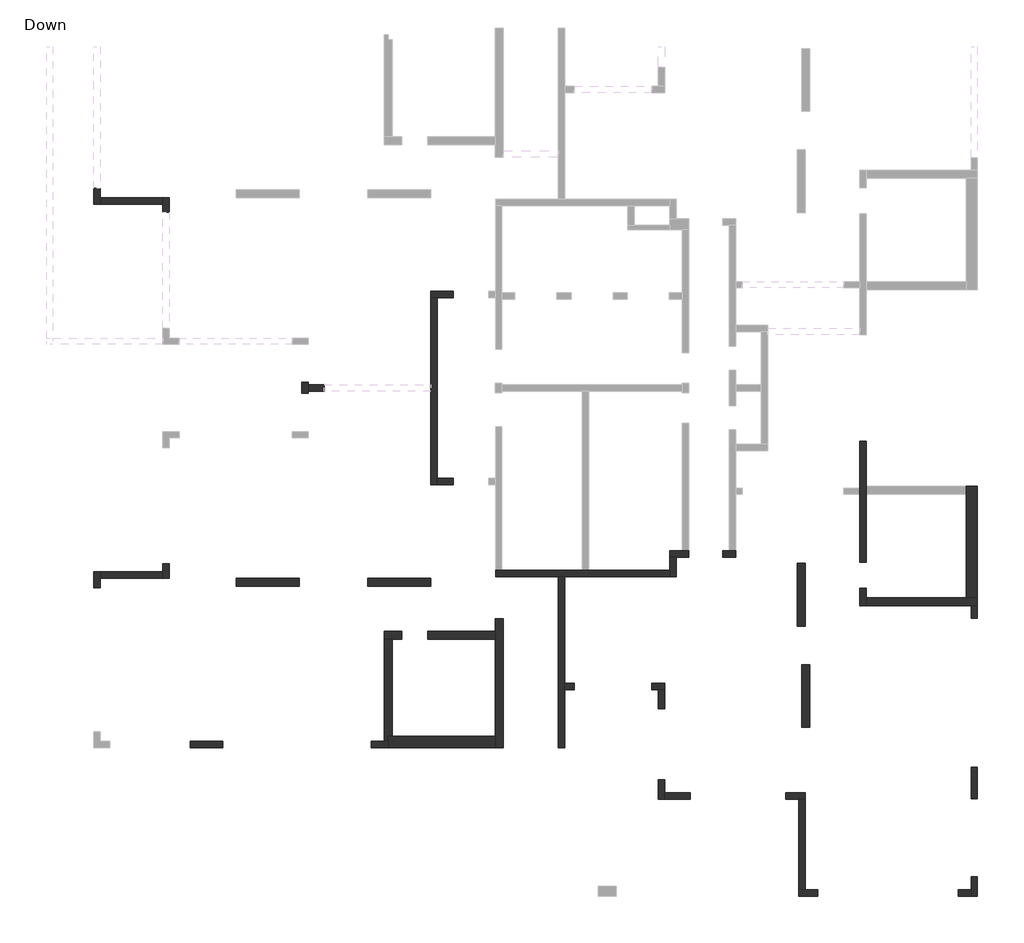
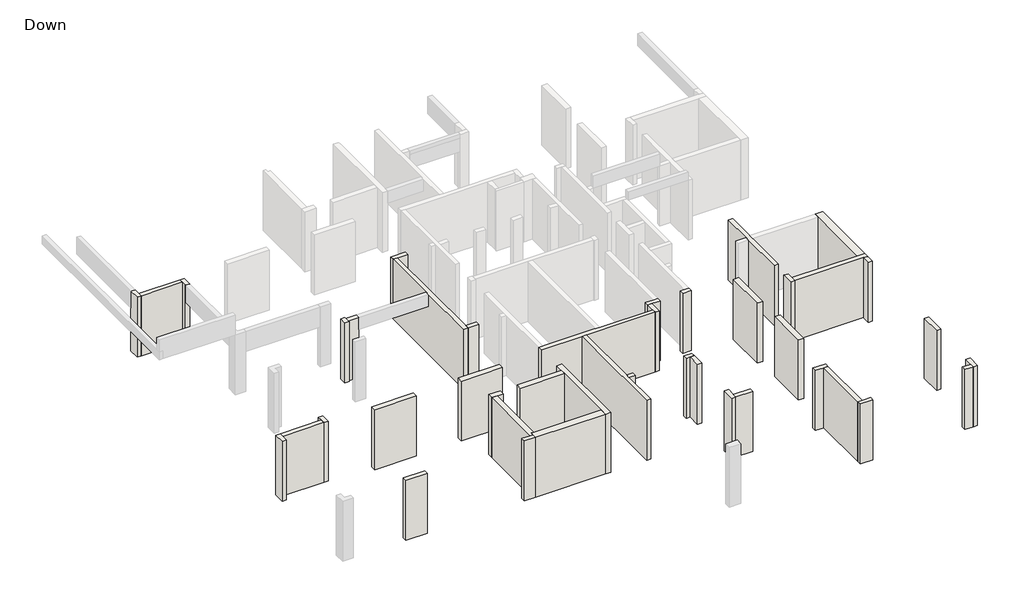
# One storey, part 1 of 3: 43 walls.
"""IFC4 building model written with IfcOpenShell, lengths in millimetres."""

from ifc_helpers import new_model, si_unit, origin, place, context, project, spatial, faceted_brep, element, save

model = new_model("IFC4")

# Units and contexts
model_context = context("Model", 3, world=origin())
ifc_project = project(units=[si_unit("LENGTHUNIT", "METRE", prefix="MILLI")], contexts=[model_context])

# Site, building, storey
site = spatial("IfcSite", under=ifc_project)
building = spatial("IfcBuilding", under=site)
storey = spatial("IfcBuildingStorey", under=building, Name="Down", Elevation=0.0)

# Walls
placement = place(None, origin())
element("IfcWall", 1, ObjectType="20", at=placement, inside=storey, context=model_context, shape_type="Brep", body=[
    faceted_brep([(-9805.5395337, 8939.7491377, 0.0), (-9805.5395337, 9386.8536298, 0.0), (-9805.5395337, 9386.8536298, 2820.0), (-9805.5395337, 9386.8536298, 3000.0), (-9805.5395337, 8939.7491377, 3000.0), (-9805.5395337, 8939.7491377, 2150.0), (-10005.5395337, 8939.7491377, 0.0), (-10005.5395337, 8939.7491377, 2150.0), (-10005.5395337, 8939.7491377, 3000.0), (-10005.5395337, 9186.8536298, 3000.0), (-10005.5395337, 9386.8536298, 3000.0), (-10005.5395337, 9386.8536298, 0.0), (-10005.5395337, 9186.8536298, 0.0)], [[[0, 1, 2, 3, 4, 5]], [[6, 7, 8, 9, 10, 11, 12]], [[1, 0, 6, 12, 11]], [[4, 3, 10, 9, 8]], [[0, 5, 4, 8, 7, 6]], [[3, 2, 1, 11, 10]]]),
])
element("IfcWall", 2, ObjectType="20", at=placement, inside=storey, context=model_context, shape_type="Brep", body=[
    faceted_brep([(-10005.5395337, 9386.8536298, 0.0), (-11954.2455884, 9386.8536298, 0.0), (-11954.2455884, 9386.8536298, 2820.0), (-11954.2455884, 9386.8536298, 3000.0), (-10005.5395337, 9386.8536298, 3000.0), (-10005.5395337, 9186.8536298, 0.0), (-10005.5395337, 9186.8536298, 2750.0), (-10005.5395337, 9186.8536298, 3000.0), (-11954.2455884, 9186.8536298, 3000.0), (-11954.2455884, 9186.8536298, 0.0)], [[[0, 1, 2, 3, 4]], [[5, 6, 7, 8, 9]], [[1, 0, 5, 9]], [[4, 3, 8, 7]], [[0, 4, 7, 6, 5]], [[3, 2, 1, 9, 8]]]),
])
element("IfcWall", 3, ObjectType="20", at=placement, inside=storey, context=model_context, shape_type="Brep", body=[
    faceted_brep([(-11954.2455884, 9186.8536298, 0.0), (-11954.2455884, 9386.8536298, 0.0), (-11954.2455884, 9686.3702314, 0.0), (-11954.2455884, 9686.3702314, 2150.0), (-11954.2455884, 9686.3702314, 3000.0), (-11954.2455884, 9386.8536298, 3000.0), (-11954.2455884, 9186.8536298, 3000.0), (-12154.2455884, 9186.8536298, 0.0), (-12154.2455884, 9186.8536298, 2750.0), (-12154.2455884, 9186.8536298, 3000.0), (-12154.2455884, 9686.3702314, 3000.0), (-12154.2455884, 9686.3702314, 2150.0), (-12154.2455884, 9686.3702314, 0.0)], [[[0, 1, 2, 3, 4, 5, 6]], [[7, 8, 9, 10, 11, 12]], [[2, 1, 0, 7, 12]], [[4, 3, 2, 12, 11, 10]], [[6, 5, 4, 10, 9]], [[0, 6, 9, 8, 7]]]),
])
element("IfcWall", 4, ObjectType="20", at=placement, inside=storey, context=model_context, shape_type="Brep", body=[
    faceted_brep([(-1004.8486157, 6491.5264814, 0.0), (-1704.8486157, 6491.5264814, 0.0), (-1704.8486157, 6491.5264814, 2820.0), (-1704.8486157, 6491.5264814, 3000.0), (-1004.8486157, 6491.5264814, 3000.0), (-1004.8486157, 6491.5264814, 2820.0), (-1004.8486157, 6291.5264814, 0.0), (-1004.8486157, 6291.5264814, 2820.0), (-1004.8486157, 6291.5264814, 3000.0), (-1504.8486157, 6291.5264814, 3000.0), (-1704.8486157, 6291.5264814, 3000.0), (-1704.8486157, 6291.5264814, 0.0), (-1504.8486157, 6291.5264814, 0.0)], [[[0, 1, 2, 3, 4, 5]], [[6, 7, 8, 9, 10, 11, 12]], [[1, 0, 6, 12, 11]], [[4, 3, 10, 9, 8]], [[0, 5, 4, 8, 7, 6]], [[3, 2, 1, 11, 10]]]),
])
element("IfcWall", 5, ObjectType="20", at=placement, inside=storey, context=model_context, shape_type="Brep", body=[
    faceted_brep([(-1704.8486157, 6291.5264814, 0.0), (-1704.8486157, 491.1895673, 0.0), (-1704.8486157, 491.1895673, 2820.0), (-1704.8486157, 491.1895673, 3000.0), (-1704.8486157, 3390.0103681, 3000.0), (-1704.8486157, 3590.0103681, 3000.0), (-1704.8486157, 6291.5264814, 3000.0), (-1504.8486157, 6291.5264814, 0.0), (-1504.8486157, 6291.5264814, 2820.0), (-1504.8486157, 6291.5264814, 3000.0), (-1504.8486157, 691.1895673, 3000.0), (-1504.8486157, 491.1895673, 3000.0), (-1504.8486157, 491.1895673, 0.0), (-1504.8486157, 691.1895673, 0.0)], [[[0, 1, 2, 3, 4, 5, 6]], [[7, 8, 9, 10, 11, 12, 13]], [[1, 0, 7, 13, 12]], [[6, 5, 4, 3, 11, 10, 9]], [[0, 6, 9, 8, 7]], [[3, 2, 1, 12, 11]]]),
])
element("IfcWall", 6, ObjectType="20", at=placement, inside=storey, context=model_context, shape_type="Brep", body=[
    faceted_brep([(-1504.8486157, 491.1895673, 0.0), (-999.8486157, 491.1895673, 0.0), (-999.8486157, 491.1895673, 2820.0), (-999.8486157, 491.1895673, 3000.0), (-1504.8486157, 491.1895673, 3000.0), (-1504.8486157, 691.1895673, 0.0), (-1504.8486157, 691.1895673, 2820.0), (-1504.8486157, 691.1895673, 3000.0), (-999.8486157, 691.1895673, 3000.0), (-999.8486157, 691.1895673, 2820.0), (-999.8486157, 691.1895673, 0.0), (-999.8486157, 688.4942548, 3000.0)], [[[0, 1, 2, 3, 4]], [[5, 6, 7, 8, 9, 10]], [[1, 0, 5, 10]], [[3, 2, 1, 10, 9, 8, 11]], [[4, 3, 11, 8, 7]], [[0, 4, 7, 6, 5]]]),
])
element("IfcWall", 7, ObjectType="20", at=placement, inside=storey, context=model_context, shape_type="Brep", body=[
    faceted_brep([(-5499.4457837, 3320.5572431, 0.0), (-5499.4457837, 3390.0103681, 0.0), (-5499.4457837, 3590.0103681, 0.0), (-5499.4457837, 3661.3116377, 0.0), (-5499.4457837, 3661.3116377, 3000.0), (-5499.4457837, 3590.0103681, 3000.0), (-5499.4457837, 3390.0103681, 3000.0), (-5499.4457837, 3320.5572431, 3000.0), (-5699.4457837, 3320.5572431, 0.0), (-5699.4457837, 3320.5572431, 3000.0), (-5699.4457837, 3661.3116377, 3000.0), (-5699.4457837, 3661.3116377, 0.0)], [[[0, 1, 2, 3, 4, 5, 6, 7]], [[8, 9, 10, 11]], [[3, 2, 1, 0, 8, 11]], [[4, 3, 11, 10]], [[7, 6, 5, 4, 10, 9]], [[0, 7, 9, 8]]]),
])
element("IfcWall", 8, ObjectType="20", at=placement, inside=storey, context=model_context, shape_type="Brep", body=[
    faceted_brep([(-5004.9145337, 3590.0103681, 0.0), (-5499.4457837, 3590.0103681, 0.0), (-5499.4457837, 3590.0103681, 2820.0), (-5499.4457837, 3590.0103681, 3000.0), (-5004.9145337, 3590.0103681, 3000.0), (-5004.9145337, 3590.0103681, 2400.0), (-5004.9145337, 3390.0103681, 0.0), (-5004.9145337, 3390.0103681, 2400.0), (-5004.9145337, 3390.0103681, 3000.0), (-5499.4457837, 3390.0103681, 3000.0), (-5499.4457837, 3390.0103681, 2820.0), (-5499.4457837, 3390.0103681, 0.0)], [[[0, 1, 2, 3, 4, 5]], [[6, 7, 8, 9, 10, 11]], [[1, 0, 6, 11]], [[4, 3, 9, 8]], [[0, 5, 4, 8, 7, 6]], [[3, 2, 1, 11, 10, 9]]]),
])
element("IfcWall", 9, ObjectType="20", at=placement, inside=storey, context=model_context, shape_type="Brep", body=[
    faceted_brep([(-10005.5395337, -1959.7284014, 0.0), (-10005.5395337, -2206.8328936, 0.0), (-10005.5395337, -2406.8328936, 0.0), (-10005.5395337, -2406.8328936, 3000.0), (-10005.5395337, -2206.8328936, 3000.0), (-10005.5395337, -1959.7284014, 3000.0), (-10005.5395337, -1959.7284014, 2150.0), (-9805.5395337, -1959.7284014, 0.0), (-9805.5395337, -1959.7284014, 2150.0), (-9805.5395337, -1959.7284014, 3000.0), (-9805.5395337, -2406.8328936, 3000.0), (-9805.5395337, -2406.8328936, 2820.0), (-9805.5395337, -2406.8328936, 0.0)], [[[0, 1, 2, 3, 4, 5, 6]], [[7, 8, 9, 10, 11, 12]], [[2, 1, 0, 7, 12]], [[5, 4, 3, 10, 9]], [[0, 6, 5, 9, 8, 7]], [[3, 2, 12, 11, 10]]]),
])
element("IfcWall", 10, ObjectType="20", at=placement, inside=storey, context=model_context, shape_type="Brep", body=[
    faceted_brep([(-10005.5395337, -2206.8328936, 0.0), (-11954.2455884, -2206.8328936, 0.0), (-11954.2455884, -2206.8328936, 3000.0), (-10005.5395337, -2206.8328936, 3000.0), (-10005.5395337, -2206.8328936, 2750.0), (-10005.5395337, -2406.8328936, 0.0), (-10005.5395337, -2406.8328936, 3000.0), (-11954.2455884, -2406.8328936, 3000.0), (-11954.2455884, -2406.8328936, 2820.0), (-11954.2455884, -2406.8328936, 0.0)], [[[0, 1, 2, 3, 4]], [[5, 6, 7, 8, 9]], [[1, 0, 5, 9]], [[3, 2, 7, 6]], [[0, 4, 3, 6, 5]], [[2, 1, 9, 8, 7]]]),
])
element("IfcWall", 11, ObjectType="20", at=placement, inside=storey, context=model_context, shape_type="Brep", body=[
    faceted_brep([(-12154.2455884, -2206.8328936, 0.0), (-12154.2455884, -2706.3494952, 0.0), (-12154.2455884, -2706.3494952, 2150.0), (-12154.2455884, -2706.3494952, 3000.0), (-12154.2455884, -2206.8328936, 3000.0), (-12154.2455884, -2206.8328936, 2750.0), (-11954.2455884, -2206.8328936, 0.0), (-11954.2455884, -2206.8328936, 3000.0), (-11954.2455884, -2406.8328936, 3000.0), (-11954.2455884, -2706.3494952, 3000.0), (-11954.2455884, -2706.3494952, 2150.0), (-11954.2455884, -2706.3494952, 0.0), (-11954.2455884, -2406.8328936, 0.0)], [[[0, 1, 2, 3, 4, 5]], [[6, 7, 8, 9, 10, 11, 12]], [[1, 0, 6, 12, 11]], [[3, 2, 1, 11, 10, 9]], [[4, 3, 9, 8, 7]], [[0, 5, 4, 7, 6]]]),
])
element("IfcWall", 12, ObjectType="20", at=placement, inside=storey, context=model_context, shape_type="Brep", body=[
    faceted_brep([(-3022.0483227, -7461.3958819, 0.0), (-3147.0483227, -7461.3958819, 0.0), (-3547.0483227, -7461.3958819, 0.0), (-3547.0483227, -7461.3958819, 2450.0), (-3547.0483227, -7461.3958819, 2820.0), (-3547.0483227, -7461.3958819, 3000.0), (-3147.0483227, -7461.3958819, 3000.0), (-3022.0483227, -7461.3958819, 3000.0), (-3022.0483227, -7661.3958819, 0.0), (-3022.0483227, -7661.3958819, 3000.0), (-3547.0483227, -7661.3958819, 3000.0), (-3547.0483227, -7661.3958819, 2450.0), (-3547.0483227, -7661.3958819, 0.0), (-3547.0483227, -7466.3958819, 3000.0)], [[[0, 1, 2, 3, 4, 5, 6, 7]], [[8, 9, 10, 11, 12]], [[2, 1, 0, 8, 12]], [[5, 4, 3, 2, 12, 11, 10, 13]], [[7, 6, 5, 13, 10, 9]], [[0, 7, 9, 8]]]),
])
element("IfcWall", 13, ObjectType="20", at=placement, inside=storey, context=model_context, shape_type="Brep", body=[
    faceted_brep([(-9154.7387524, -7661.3958819, 0.0), (-8149.7387524, -7661.3958819, 0.0), (-8149.7387524, -7661.3958819, 2450.0), (-8149.7387524, -7661.3958819, 3000.0), (-9154.7387524, -7661.3958819, 3000.0), (-9154.7387524, -7661.3958819, 2450.0), (-9154.7387524, -7461.3958819, 0.0), (-9154.7387524, -7461.3958819, 2450.0), (-9154.7387524, -7461.3958819, 2820.0), (-9154.7387524, -7461.3958819, 3000.0), (-8149.7387524, -7461.3958819, 3000.0), (-8149.7387524, -7461.3958819, 2820.0), (-8149.7387524, -7461.3958819, 2450.0), (-8149.7387524, -7461.3958819, 0.0), (-8149.7387524, -7466.3958819, 3000.0), (-9154.7387524, -7466.3958819, 3000.0)], [[[0, 1, 2, 3, 4, 5]], [[6, 7, 8, 9, 10, 11, 12, 13]], [[1, 0, 6, 13]], [[3, 2, 1, 13, 12, 11, 10, 14]], [[4, 3, 14, 10, 9, 15]], [[0, 5, 4, 15, 9, 8, 7, 6]]]),
])
element("IfcWall", 14, ObjectType="20", at=placement, inside=storey, context=model_context, shape_type="Brep", body=[
    faceted_brep([(2446.4257984, -7661.3958819, 0.0), (2446.4257984, -5860.2777178, 0.0), (2446.4257984, -5660.2777178, 0.0), (2446.4257984, -2357.0550616, 0.0), (2446.4257984, -2357.0550616, 2820.0), (2446.4257984, -2357.0550616, 3000.0), (2446.4257984, -5660.2777178, 3000.0), (2446.4257984, -5860.2777178, 3000.0), (2446.4257984, -7661.3958819, 3000.0), (2446.4257984, -7661.3958819, 2750.0), (2246.4257984, -7661.3958819, 0.0), (2246.4257984, -7661.3958819, 2750.0), (2246.4257984, -7661.3958819, 3000.0), (2246.4257984, -7461.3958819, 3000.0), (2246.4257984, -3861.3299639, 3000.0), (2246.4257984, -3661.3299639, 3000.0), (2246.4257984, -2357.0550616, 3000.0), (2246.4257984, -2357.0550616, 2820.0), (2246.4257984, -2357.0550616, 0.0)], [[[0, 1, 2, 3, 4, 5, 6, 7, 8, 9]], [[10, 11, 12, 13, 14, 15, 16, 17, 18]], [[3, 2, 1, 0, 10, 18]], [[8, 7, 6, 5, 16, 15, 14, 13, 12]], [[0, 9, 8, 12, 11, 10]], [[5, 4, 3, 18, 17, 16]]]),
])
element("IfcWall", 15, ObjectType="20", at=placement, inside=storey, context=model_context, shape_type="Brep", body=[
    faceted_brep([(2745.6201343, -5660.2777178, 0.0), (2446.4257984, -5660.2777178, 0.0), (2446.4257984, -5660.2777178, 2820.0), (2446.4257984, -5660.2777178, 3000.0), (2745.6201343, -5660.2777178, 3000.0), (2745.6201343, -5660.2777178, 2820.0), (2745.6201343, -5660.2777178, 2150.0), (2745.6201343, -5860.2777178, 0.0), (2745.6201343, -5860.2777178, 2150.0), (2745.6201343, -5860.2777178, 3000.0), (2446.4257984, -5860.2777178, 3000.0), (2446.4257984, -5860.2777178, 0.0), (2745.6201343, -5665.2777178, 3000.0)], [[[0, 1, 2, 3, 4, 5, 6]], [[7, 8, 9, 10, 11]], [[1, 0, 7, 11]], [[4, 3, 10, 9, 12]], [[0, 6, 5, 4, 12, 9, 8, 7]], [[3, 2, 1, 11, 10]]]),
])
element("IfcWall", 16, ObjectType="20", at=placement, inside=storey, context=model_context, shape_type="Brep", body=[
    faceted_brep([(5152.6049976, -5860.2777178, 0.0), (5345.4492359, -5860.2777178, 0.0), (5545.4492359, -5860.2777178, 0.0), (5545.4492359, -5860.2777178, 3000.0), (5345.4492359, -5860.2777178, 3000.0), (5152.6049976, -5860.2777178, 3000.0), (5152.6049976, -5860.2777178, 2150.0), (5152.6049976, -5660.2777178, 0.0), (5152.6049976, -5660.2777178, 2150.0), (5152.6049976, -5660.2777178, 2820.0), (5152.6049976, -5660.2777178, 3000.0), (5545.4492359, -5660.2777178, 3000.0), (5545.4492359, -5660.2777178, 2820.0), (5545.4492359, -5660.2777178, 0.0), (5152.6049976, -5665.2777178, 3000.0)], [[[0, 1, 2, 3, 4, 5, 6]], [[7, 8, 9, 10, 11, 12, 13]], [[2, 1, 0, 7, 13]], [[5, 4, 3, 11, 10, 14]], [[0, 6, 5, 14, 10, 9, 8, 7]], [[3, 2, 13, 12, 11]]]),
])
element("IfcWall", 17, ObjectType="20", at=placement, inside=storey, context=model_context, shape_type="Brep", body=[
    faceted_brep([(5345.4492359, -5860.2777178, 0.0), (5345.4492359, -6456.8182452, 0.0), (5345.4492359, -6456.8182452, 2150.0), (5345.4492359, -6456.8182452, 3000.0), (5345.4492359, -5860.2777178, 3000.0), (5345.4492359, -5860.2777178, 2750.0), (5545.4492359, -5860.2777178, 0.0), (5545.4492359, -5860.2777178, 3000.0), (5545.4492359, -6456.8182452, 3000.0), (5545.4492359, -6456.8182452, 2150.0), (5545.4492359, -6456.8182452, 0.0)], [[[0, 1, 2, 3, 4, 5]], [[6, 7, 8, 9, 10]], [[1, 0, 6, 10]], [[3, 2, 1, 10, 9, 8]], [[4, 3, 8, 7]], [[0, 5, 4, 7, 6]]]),
])
element("IfcWall", 18, ObjectType="20", at=placement, inside=storey, context=model_context, shape_type="Brep", body=[
    faceted_brep([(5345.4492359, -8661.9549639, 0.0), (5345.4492359, -9261.9549639, 0.0), (5345.4492359, -9261.9549639, 2750.0), (5345.4492359, -9261.9549639, 3000.0), (5345.4492359, -8661.9549639, 3000.0), (5345.4492359, -8661.9549639, 2150.0), (5545.4492359, -8661.9549639, 0.0), (5545.4492359, -8661.9549639, 2150.0), (5545.4492359, -8661.9549639, 3000.0), (5545.4492359, -9061.9549639, 3000.0), (5545.4492359, -9261.9549639, 3000.0), (5545.4492359, -9261.9549639, 0.0), (5545.4492359, -9061.9549639, 0.0)], [[[0, 1, 2, 3, 4, 5]], [[6, 7, 8, 9, 10, 11, 12]], [[1, 0, 6, 12, 11]], [[4, 3, 10, 9, 8]], [[0, 5, 4, 8, 7, 6]], [[3, 2, 1, 11, 10]]]),
])
element("IfcWall", 19, ObjectType="20", at=placement, inside=storey, context=model_context, shape_type="Brep", body=[
    faceted_brep([(5545.4492359, -9261.9549639, 0.0), (6350.1123218, -9261.9549639, 0.0), (6350.1123218, -9261.9549639, 2150.0), (6350.1123218, -9261.9549639, 3000.0), (5545.4492359, -9261.9549639, 3000.0), (5545.4492359, -9061.9549639, 0.0), (5545.4492359, -9061.9549639, 2820.0), (5545.4492359, -9061.9549639, 3000.0), (6350.1123218, -9061.9549639, 3000.0), (6350.1123218, -9061.9549639, 2150.0), (6350.1123218, -9061.9549639, 0.0)], [[[0, 1, 2, 3, 4]], [[5, 6, 7, 8, 9, 10]], [[1, 0, 5, 10]], [[3, 2, 1, 10, 9, 8]], [[4, 3, 8, 7]], [[0, 4, 7, 6, 5]]]),
])
element("IfcWall", 20, ObjectType="20", at=placement, inside=storey, context=model_context, shape_type="Brep", body=[
    faceted_brep([(9302.4292163, -9261.9354327, 0.0), (9702.4292163, -9261.9354327, 0.0), (9902.4292163, -9261.9354327, 0.0), (9902.4292163, -9261.9354327, 3000.0), (9702.4292163, -9261.9354327, 3000.0), (9302.4292163, -9261.9354327, 3000.0), (9302.4292163, -9061.9354327, 0.0), (9302.4292163, -9061.9354327, 3000.0), (9902.4292163, -9061.9354327, 3000.0), (9902.4292163, -9061.9354327, 2820.0), (9902.4292163, -9061.9354327, 0.0)], [[[0, 1, 2, 3, 4, 5]], [[6, 7, 8, 9, 10]], [[2, 1, 0, 6, 10]], [[5, 4, 3, 8, 7]], [[0, 5, 7, 6]], [[3, 2, 10, 9, 8]]]),
])
element("IfcWall", 21, ObjectType="20", at=placement, inside=storey, context=model_context, shape_type="Brep", body=[
    faceted_brep([(9702.4292163, -9261.9354327, 0.0), (9702.4292163, -12061.3104327, 0.0), (9702.4292163, -12061.3104327, 3000.0), (9702.4292163, -9261.9354327, 3000.0), (9702.4292163, -9261.9354327, 2750.0), (9902.4292163, -9261.9354327, 0.0), (9902.4292163, -9261.9354327, 3000.0), (9902.4292163, -12061.3104327, 3000.0), (9902.4292163, -12061.3104327, 2820.0), (9902.4292163, -12061.3104327, 0.0)], [[[0, 1, 2, 3, 4]], [[5, 6, 7, 8, 9]], [[1, 0, 5, 9]], [[3, 2, 7, 6]], [[0, 4, 3, 6, 5]], [[2, 1, 9, 8, 7]]]),
])
element("IfcWall", 22, ObjectType="20", at=placement, inside=storey, context=model_context, shape_type="Brep", body=[
    faceted_brep([(9702.4292163, -12261.3104327, 0.0), (10302.4292163, -12261.3104327, 0.0), (10302.4292163, -12261.3104327, 2400.0), (10302.4292163, -12261.3104327, 3000.0), (9702.4292163, -12261.3104327, 3000.0), (9702.4292163, -12261.3104327, 2750.0), (9702.4292163, -12061.3104327, 0.0), (9702.4292163, -12061.3104327, 3000.0), (9902.4292163, -12061.3104327, 3000.0), (10302.4292163, -12061.3104327, 3000.0), (10302.4292163, -12061.3104327, 2820.0), (10302.4292163, -12061.3104327, 2400.0), (10302.4292163, -12061.3104327, 0.0), (9902.4292163, -12061.3104327, 0.0), (10302.4292163, -12066.3104327, 3000.0)], [[[0, 1, 2, 3, 4, 5]], [[6, 7, 8, 9, 10, 11, 12, 13]], [[1, 0, 6, 13, 12]], [[3, 2, 1, 12, 11, 10, 9, 14]], [[4, 3, 14, 9, 8, 7]], [[0, 5, 4, 7, 6]]]),
])
element("IfcWall", 23, ObjectType="20", at=placement, inside=storey, context=model_context, shape_type="Brep", body=[
    faceted_brep([(14652.4902515, -12261.3104327, 0.0), (15047.1826343, -12261.3104327, 0.0), (15047.1826343, -12261.3104327, 3000.0), (14652.4902515, -12261.3104327, 3000.0), (14652.4902515, -12261.3104327, 2400.0), (14652.4902515, -12061.3104327, 0.0), (14652.4902515, -12061.3104327, 2400.0), (14652.4902515, -12061.3104327, 2820.0), (14652.4902515, -12061.3104327, 3000.0), (15047.1826343, -12061.3104327, 3000.0), (15047.1826343, -12061.3104327, 2820.0), (15047.1826343, -12061.3104327, 0.0), (14652.4902515, -12066.3104327, 3000.0)], [[[0, 1, 2, 3, 4]], [[5, 6, 7, 8, 9, 10, 11]], [[1, 0, 5, 11]], [[3, 2, 9, 8, 12]], [[0, 4, 3, 12, 8, 7, 6, 5]], [[2, 1, 11, 10, 9]]]),
])
element("IfcWall", 24, ObjectType="20", at=placement, inside=storey, context=model_context, shape_type="Brep", body=[
    faceted_brep([(15247.1826343, -12261.3104327, 0.0), (15247.1826343, -11661.3104327, 0.0), (15247.1826343, -11661.3104327, 2400.0), (15247.1826343, -11661.3104327, 3000.0), (15247.1826343, -12261.3104327, 3000.0), (15047.1826343, -12261.3104327, 0.0), (15047.1826343, -12261.3104327, 3000.0), (15047.1826343, -12061.3104327, 3000.0), (15047.1826343, -11661.3104327, 3000.0), (15047.1826343, -11661.3104327, 2400.0), (15047.1826343, -11661.3104327, 0.0), (15047.1826343, -12061.3104327, 0.0)], [[[0, 1, 2, 3, 4]], [[5, 6, 7, 8, 9, 10, 11]], [[1, 0, 5, 11, 10]], [[3, 2, 1, 10, 9, 8]], [[4, 3, 8, 7, 6]], [[0, 4, 6, 5]]]),
])
element("IfcWall", 25, ObjectType="20", at=placement, inside=storey, context=model_context, shape_type="Brep", body=[
    faceted_brep([(15247.1826343, -9252.3065264, 0.0), (15247.1826343, -8260.429085, 0.0), (15247.1826343, -8260.429085, 2400.0), (15247.1826343, -8260.429085, 3000.0), (15247.1826343, -9252.3065264, 3000.0), (15247.1826343, -9252.3065264, 2400.0), (15047.1826343, -9252.3065264, 0.0), (15047.1826343, -9252.3065264, 2400.0), (15047.1826343, -9252.3065264, 3000.0), (15047.1826343, -8260.429085, 3000.0), (15047.1826343, -8260.429085, 2400.0), (15047.1826343, -8260.429085, 0.0)], [[[0, 1, 2, 3, 4, 5]], [[6, 7, 8, 9, 10, 11]], [[1, 0, 6, 11]], [[3, 2, 1, 11, 10, 9]], [[4, 3, 9, 8]], [[0, 5, 4, 8, 7, 6]]]),
])
element("IfcWall", 26, ObjectType="20", at=placement, inside=storey, context=model_context, shape_type="Brep", body=[
    faceted_brep([(15247.1826343, -3654.8187334, 0.0), (15247.1826343, -3259.804085, 0.0), (15247.1826343, -3259.804085, 3000.0), (15247.1826343, -3654.8187334, 3000.0), (15247.1826343, -3654.8187334, 2400.0), (15047.1826343, -3654.8187334, 0.0), (15047.1826343, -3654.8187334, 2400.0), (15047.1826343, -3654.8187334, 3000.0), (15047.1826343, -3259.804085, 3000.0), (15047.1826343, -3259.804085, 0.0)], [[[0, 1, 2, 3, 4]], [[5, 6, 7, 8, 9]], [[1, 0, 5, 9]], [[3, 2, 8, 7]], [[0, 4, 3, 7, 6, 5]], [[2, 1, 9, 8]]]),
])
element("IfcWall", 27, ObjectType="20", at=placement, inside=storey, context=model_context, shape_type="Brep", body=[
    faceted_brep([(11796.5527515, -3259.804085, 0.0), (11796.5527515, -3009.804085, 0.0), (11796.5527515, -2710.6903155, 0.0), (11796.5527515, -2710.6903155, 3000.0), (11796.5527515, -3009.804085, 3000.0), (11796.5527515, -3259.804085, 3000.0), (11596.5527515, -3259.804085, 0.0), (11596.5527515, -3259.804085, 2820.0), (11596.5527515, -3259.804085, 3000.0), (11596.5527515, -2710.6903155, 3000.0), (11596.5527515, -2710.6903155, 0.0)], [[[0, 1, 2, 3, 4, 5]], [[6, 7, 8, 9, 10]], [[2, 1, 0, 6, 10]], [[3, 2, 10, 9]], [[5, 4, 3, 9, 8]], [[0, 5, 8, 7, 6]]]),
])
element("IfcWall", 28, ObjectType="20", at=placement, inside=storey, context=model_context, shape_type="Brep", body=[
    faceted_brep([(11796.5527515, -1909.8089678, 0.0), (11796.5527515, 188.5748212, 0.0), (11796.5527515, 438.5748212, 0.0), (11796.5527515, 1845.1910322, 0.0), (11796.5527515, 1845.1910322, 3000.0), (11796.5527515, 438.5748212, 3000.0), (11796.5527515, 188.5748212, 3000.0), (11796.5527515, -1909.8089678, 3000.0), (11796.5527515, -1909.8089678, 2820.0), (11596.5527515, -1909.8089678, 0.0), (11596.5527515, -1909.8089678, 2820.0), (11596.5527515, -1909.8089678, 3000.0), (11596.5527515, 188.6553877, 3000.0), (11596.5527515, 388.6553877, 3000.0), (11596.5527515, 1845.1910322, 3000.0), (11596.5527515, 1845.1910322, 2820.0), (11596.5527515, 1845.1910322, 0.0), (11596.5527515, 388.6553877, 0.0), (11596.5527515, 188.6553877, 0.0)], [[[0, 1, 2, 3, 4, 5, 6, 7, 8]], [[9, 10, 11, 12, 13, 14, 15, 16, 17, 18]], [[3, 2, 1, 0, 9, 18, 17, 16]], [[4, 3, 16, 15, 14]], [[7, 6, 5, 4, 14, 13, 12, 11]], [[0, 8, 7, 11, 10, 9]]]),
])
element("IfcWall", 29, ObjectType="20", at=placement, inside=storey, context=model_context, shape_type="Brep", body=[
    faceted_brep([(5901.4257984, -2357.0550616, 0.0), (5901.4257984, -1759.7284014, 0.0), (5901.4257984, -1759.7284014, 2820.0), (5901.4257984, -1759.7284014, 3000.0), (5901.4257984, -2357.0550616, 3000.0), (5901.4257984, -2357.0550616, 2820.0), (5701.4257984, -2357.0550616, 0.0), (5701.4257984, -2357.0550616, 3000.0), (5701.4257984, -2157.0550616, 3000.0), (5701.4257984, -1759.7284014, 3000.0), (5701.4257984, -1759.7284014, 0.0), (5701.4257984, -2157.0550616, 0.0)], [[[0, 1, 2, 3, 4, 5]], [[6, 7, 8, 9, 10, 11]], [[1, 0, 6, 11, 10]], [[4, 3, 9, 8, 7]], [[3, 2, 1, 10, 9]], [[0, 5, 4, 7, 6]]]),
])
element("IfcWall", 30, ObjectType="20", at=placement, inside=storey, context=model_context, shape_type="Brep", body=[
    faceted_brep([(5701.4257984, -2157.0550616, 0.0), (3197.0654468, -2157.0550616, 0.0), (2997.0654468, -2157.0550616, 0.0), (506.4257984, -2157.0550616, 0.0), (306.4257984, -2157.0550616, 0.0), (306.4257984, -2157.0550616, 3000.0), (506.4257984, -2157.0550616, 3000.0), (2997.0654468, -2157.0550616, 3000.0), (3197.0654468, -2157.0550616, 3000.0), (5701.4257984, -2157.0550616, 3000.0), (5701.4257984, -2357.0550616, 0.0), (5701.4257984, -2357.0550616, 3000.0), (2446.4257984, -2357.0550616, 3000.0), (2246.4257984, -2357.0550616, 3000.0), (306.4257984, -2357.0550616, 3000.0), (306.4257984, -2357.0550616, 2820.0), (306.4257984, -2357.0550616, 0.0), (2246.4257984, -2357.0550616, 0.0), (2446.4257984, -2357.0550616, 0.0)], [[[0, 1, 2, 3, 4, 5, 6, 7, 8, 9]], [[10, 11, 12, 13, 14, 15, 16, 17, 18]], [[4, 3, 2, 1, 0, 10, 18, 17, 16]], [[9, 8, 7, 6, 5, 14, 13, 12, 11]], [[5, 4, 16, 15, 14]], [[0, 9, 11, 10]]]),
])
element("IfcWall", 31, ObjectType="20", at=placement, inside=storey, context=model_context, shape_type="Brep", body=[
    faceted_brep([(7351.2304859, -1760.3729327, 0.0), (7751.2304859, -1760.3729327, 0.0), (7751.2304859, -1760.3729327, 2820.0), (7751.2304859, -1760.3729327, 3000.0), (7351.2304859, -1760.3729327, 3000.0), (7351.2304859, -1760.3729327, 2820.0), (7351.2304859, -1560.3729327, 0.0), (7351.2304859, -1560.3729327, 2820.0), (7351.2304859, -1560.3729327, 3000.0), (7551.2304859, -1560.3729327, 3000.0), (7751.2304859, -1560.3729327, 3000.0), (7751.2304859, -1560.3729327, 0.0), (7551.2304859, -1560.3729327, 0.0), (7351.2304859, -1759.7284014, 3000.0)], [[[0, 1, 2, 3, 4, 5]], [[6, 7, 8, 9, 10, 11, 12]], [[1, 0, 6, 12, 11]], [[4, 3, 10, 9, 8, 13]], [[0, 5, 4, 13, 8, 7, 6]], [[3, 2, 1, 11, 10]]]),
])
element("IfcWall", 32, ObjectType="20", at=placement, inside=storey, context=model_context, shape_type="Brep", body=[
    faceted_brep([(5701.4257984, -1759.7284014, 0.0), (5901.4257984, -1759.7284014, 0.0), (6296.4111499, -1759.7284014, 0.0), (6296.4111499, -1759.7284014, 2820.0), (6296.4111499, -1759.7284014, 3000.0), (5901.4257984, -1759.7284014, 3000.0), (5701.4257984, -1759.7284014, 3000.0), (5701.4257984, -1559.7284014, 0.0), (5701.4257984, -1559.7284014, 3000.0), (6096.4111499, -1559.7284014, 3000.0), (6296.4111499, -1559.7284014, 3000.0), (6296.4111499, -1559.7284014, 0.0), (6096.4111499, -1559.7284014, 0.0)], [[[0, 1, 2, 3, 4, 5, 6]], [[7, 8, 9, 10, 11, 12]], [[2, 1, 0, 7, 12, 11]], [[6, 5, 4, 10, 9, 8]], [[0, 6, 8, 7]], [[4, 3, 2, 11, 10]]]),
])
element("IfcWall", 33, ObjectType="25", at=placement, inside=storey, context=model_context, shape_type="Brep", body=[
    faceted_brep([(-7730.9496899, -2661.1737139, 0.0), (-5784.0917798, -2661.1737139, 0.0), (-5784.0917798, -2661.1737139, 2820.0), (-5784.0917798, -2661.1737139, 3000.0), (-7730.9496899, -2661.1737139, 3000.0), (-7730.9496899, -2661.1737139, 2820.0), (-7730.9496899, -2411.1737139, 0.0), (-7730.9496899, -2411.1737139, 2820.0), (-7730.9496899, -2411.1737139, 3000.0), (-5784.0917798, -2411.1737139, 3000.0), (-5784.0917798, -2411.1737139, 2820.0), (-5784.0917798, -2411.1737139, 0.0)], [[[0, 1, 2, 3, 4, 5]], [[6, 7, 8, 9, 10, 11]], [[1, 0, 6, 11]], [[3, 2, 1, 11, 10, 9]], [[4, 3, 9, 8]], [[0, 5, 4, 8, 7, 6]]]),
])
element("IfcWall", 34, ObjectType="25", at=placement, inside=storey, context=model_context, shape_type="Brep", body=[
    faceted_brep([(-3648.408186, -2661.1737139, 0.0), (-1703.720686, -2661.1737139, 0.0), (-1703.720686, -2661.1737139, 2820.0), (-1703.720686, -2661.1737139, 3000.0), (-3648.408186, -2661.1737139, 3000.0), (-3648.408186, -2661.1737139, 2820.0), (-3648.408186, -2411.1737139, 0.0), (-3648.408186, -2411.1737139, 2820.0), (-3648.408186, -2411.1737139, 3000.0), (-1703.720686, -2411.1737139, 3000.0), (-1703.720686, -2411.1737139, 2820.0), (-1703.720686, -2411.1737139, 0.0)], [[[0, 1, 2, 3, 4, 5]], [[6, 7, 8, 9, 10, 11]], [[1, 0, 6, 11]], [[3, 2, 1, 11, 10, 9]], [[4, 3, 9, 8]], [[0, 5, 4, 8, 7, 6]]]),
])
element("IfcWall", 35, ObjectType="25", at=placement, inside=storey, context=model_context, shape_type="Brep", body=[
    faceted_brep([(-1797.0483227, -4305.6854327, 0.0), (292.9516773, -4305.6854327, 0.0), (292.9516773, -4305.6854327, 2820.0), (292.9516773, -4305.6854327, 3000.0), (-1797.0483227, -4305.6854327, 3000.0), (-1797.0483227, -4305.6854327, 2820.0), (-1797.0483227, -4055.6854327, 0.0), (-1797.0483227, -4055.6854327, 2820.0), (-1797.0483227, -4055.6854327, 3000.0), (292.9516773, -4055.6854327, 3000.0), (292.9516773, -4055.6854327, 2820.0), (292.9516773, -4055.6854327, 0.0)], [[[0, 1, 2, 3, 4, 5]], [[6, 7, 8, 9, 10, 11]], [[1, 0, 6, 11]], [[4, 3, 9, 8]], [[0, 5, 4, 8, 7, 6]], [[3, 2, 1, 11, 10, 9]]]),
])
element("IfcWall", 36, ObjectType="25", at=placement, inside=storey, context=model_context, shape_type="Brep", body=[
    faceted_brep([(292.9516773, -3661.3299639, 0.0), (292.9516773, -4055.6854327, 0.0), (292.9516773, -4305.6854327, 0.0), (292.9516773, -7311.3958819, 0.0), (292.9516773, -7661.3958819, 0.0), (292.9516773, -7661.3958819, 3000.0), (292.9516773, -7311.3958819, 3000.0), (292.9516773, -4305.6854327, 3000.0), (292.9516773, -4055.6854327, 3000.0), (292.9516773, -3661.3299639, 3000.0), (292.9516773, -3661.3299639, 2820.0), (542.9516773, -3661.3299639, 0.0), (542.9516773, -3661.3299639, 3000.0), (542.9516773, -3861.3299639, 3000.0), (542.9516773, -7461.3958819, 3000.0), (542.9516773, -7661.3958819, 3000.0), (542.9516773, -7661.3958819, 2600.0), (542.9516773, -7661.3958819, 0.0)], [[[0, 1, 2, 3, 4, 5, 6, 7, 8, 9, 10]], [[11, 12, 13, 14, 15, 16, 17]], [[4, 3, 2, 1, 0, 11, 17]], [[9, 8, 7, 6, 5, 15, 14, 13, 12]], [[0, 10, 9, 12, 11]], [[5, 4, 17, 16, 15]]]),
])
element("IfcWall", 37, ObjectType="25", at=placement, inside=storey, context=model_context, shape_type="Brep", body=[
    faceted_brep([(-2897.0483227, -7311.3958819, 0.0), (-2897.0483227, -4305.6854327, 0.0), (-2897.0483227, -4305.6854327, 2820.0), (-2897.0483227, -4305.6854327, 3000.0), (-2897.0483227, -7311.3958819, 3000.0), (-2897.0483227, -7311.3958819, 2820.0), (-3147.0483227, -7461.3958819, 0.0), (-3147.0483227, -7461.3958819, 2820.0), (-3147.0483227, -7461.3958819, 3000.0), (-3147.0483227, -4305.6854327, 3000.0), (-3147.0483227, -4305.6854327, 0.0), (-3022.0483227, -7311.3958819, 0.0), (-3022.0483227, -7461.3958819, 0.0), (-3022.0483227, -7461.3958819, 3000.0), (-3022.0483227, -7311.3958819, 3000.0)], [[[0, 1, 2, 3, 4, 5]], [[6, 7, 8, 9, 10]], [[1, 0, 11, 12, 6, 10]], [[4, 3, 9, 8, 13, 14]], [[0, 5, 4, 14, 11]], [[14, 13, 12, 11]], [[13, 8, 7, 6, 12]], [[3, 2, 1, 10, 9]]]),
])
element("IfcWall", 38, ObjectType="25", at=placement, inside=storey, context=model_context, shape_type="Brep", body=[
    faceted_brep([(-3147.0483227, -4305.6854327, 0.0), (-2897.0483227, -4305.6854327, 0.0), (-2602.0483227, -4305.6854327, 0.0), (-2602.0483227, -4305.6854327, 2820.0), (-2602.0483227, -4305.6854327, 3000.0), (-2897.0483227, -4305.6854327, 3000.0), (-3147.0483227, -4305.6854327, 3000.0), (-3147.0483227, -4055.6854327, 0.0), (-3147.0483227, -4055.6854327, 2820.0), (-3147.0483227, -4055.6854327, 3000.0), (-2602.0483227, -4055.6854327, 3000.0), (-2602.0483227, -4055.6854327, 2820.0), (-2602.0483227, -4055.6854327, 0.0)], [[[0, 1, 2, 3, 4, 5, 6]], [[7, 8, 9, 10, 11, 12]], [[2, 1, 0, 7, 12]], [[4, 3, 2, 12, 11, 10]], [[6, 5, 4, 10, 9]], [[0, 6, 9, 8, 7]]]),
])
element("IfcWall", 39, ObjectType="25", at=placement, inside=storey, context=model_context, shape_type="Brep", body=[
    faceted_brep([(10046.8798999, -7025.4657061, 0.0), (10046.8798999, -5082.9486163, 0.0), (10046.8798999, -5082.9486163, 2820.0), (10046.8798999, -5082.9486163, 3000.0), (10046.8798999, -7025.4657061, 3000.0), (10046.8798999, -7025.4657061, 2820.0), (9796.8798999, -7025.4657061, 0.0), (9796.8798999, -7025.4657061, 2820.0), (9796.8798999, -7025.4657061, 3000.0), (9796.8798999, -5082.9486163, 3000.0), (9796.8798999, -5082.9486163, 2820.0), (9796.8798999, -5082.9486163, 0.0)], [[[0, 1, 2, 3, 4, 5]], [[6, 7, 8, 9, 10, 11]], [[1, 0, 6, 11]], [[3, 2, 1, 11, 10, 9]], [[4, 3, 9, 8]], [[0, 5, 4, 8, 7, 6]]]),
])
element("IfcWall", 40, ObjectType="25", at=placement, inside=storey, context=model_context, shape_type="Brep", body=[
    faceted_brep([(9906.2060718, -3891.3934405, 0.0), (9906.2060718, -1940.19471, 0.0), (9906.2060718, -1940.19471, 2820.0), (9906.2060718, -1940.19471, 3000.0), (9906.2060718, -3891.3934405, 3000.0), (9906.2060718, -3891.3934405, 2820.0), (9656.2060718, -3891.3934405, 0.0), (9656.2060718, -3891.3934405, 2820.0), (9656.2060718, -3891.3934405, 3000.0), (9656.2060718, -1940.19471, 3000.0), (9656.2060718, -1940.19471, 2820.0), (9656.2060718, -1940.19471, 0.0)], [[[0, 1, 2, 3, 4, 5]], [[6, 7, 8, 9, 10, 11]], [[1, 0, 6, 11]], [[3, 2, 1, 11, 10, 9]], [[4, 3, 9, 8]], [[0, 5, 4, 8, 7, 6]]]),
])
element("IfcWall", 41, ObjectType="25", at=placement, inside=storey, context=model_context, shape_type="Brep", body=[
    faceted_brep([(11796.5527515, -3259.804085, 0.0), (15047.1826343, -3259.804085, 0.0), (15247.1826343, -3259.804085, 0.0), (15247.1826343, -3259.804085, 3000.0), (15047.1826343, -3259.804085, 3000.0), (11796.5527515, -3259.804085, 3000.0), (11796.5527515, -3009.804085, 0.0), (11796.5527515, -3009.804085, 2820.0), (11796.5527515, -3009.804085, 3000.0), (14897.1826343, -3009.804085, 3000.0), (15247.1826343, -3009.804085, 3000.0), (15247.1826343, -3009.804085, 0.0), (14897.1826343, -3009.804085, 0.0)], [[[0, 1, 2, 3, 4, 5]], [[6, 7, 8, 9, 10, 11, 12]], [[2, 1, 0, 6, 12, 11]], [[5, 4, 3, 10, 9, 8]], [[3, 2, 11, 10]], [[0, 5, 8, 7, 6]]]),
])
element("IfcWall", 42, ObjectType="35", at=placement, inside=storey, context=model_context, shape_type="Brep", body=[
    faceted_brep([(292.9516773, -7311.3958819, 0.0), (-2897.0483227, -7311.3958819, 0.0), (-3022.0483227, -7311.3958819, 0.0), (-3022.0483227, -7311.3958819, 3000.0), (-2897.0483227, -7311.3958819, 3000.0), (292.9516773, -7311.3958819, 3000.0), (292.9516773, -7311.3958819, 2820.0), (292.9516773, -7661.3958819, 0.0), (292.9516773, -7661.3958819, 3000.0), (-3022.0483227, -7661.3958819, 3000.0), (-3022.0483227, -7661.3958819, 0.0), (-3022.0483227, -7461.3958819, 0.0), (-3022.0483227, -7461.3958819, 3000.0)], [[[0, 1, 2, 3, 4, 5, 6]], [[7, 8, 9, 10]], [[2, 1, 0, 7, 10, 11]], [[3, 2, 11, 10, 9, 12]], [[5, 4, 3, 12, 9, 8]], [[0, 6, 5, 8, 7]]]),
])
element("IfcWall", 43, ObjectType="35", at=placement, inside=storey, context=model_context, shape_type="Brep", body=[
    faceted_brep([(15247.1826343, -3009.804085, 0.0), (15247.1826343, 438.5748212, 0.0), (15247.1826343, 438.5748212, 3000.0), (15247.1826343, -3009.804085, 3000.0), (14897.1826343, -3009.804085, 0.0), (14897.1826343, -3009.804085, 2820.0), (14897.1826343, -3009.804085, 3000.0), (14897.1826343, 188.5748212, 3000.0), (14897.1826343, 438.5748212, 3000.0), (14897.1826343, 438.5748212, 0.0), (14897.1826343, 188.5748212, 0.0)], [[[0, 1, 2, 3]], [[4, 5, 6, 7, 8, 9, 10]], [[1, 0, 4, 10, 9]], [[3, 2, 8, 7, 6]], [[0, 3, 6, 5, 4]], [[2, 1, 9, 8]]]),
])

save(model, "model.ifc")

# Revit data of these elements
# Project information
#   Project Issue Date = "Issue Date"
#   Project Status = "Project Status"
#   Client Name = "לקוח"
#   Project Address = "Enter address here"
#   Project Name = "Project 017"
#   Project Number = "מספר פרויקט"
# Type "20"
#   Layers, outside or top first: 20 cm "Concrete" (function 1)
# Type "25"
#   Layers, outside or top first: 25 cm "Concrete" (function 1)
# Type "35"
#   Layers, outside or top first: 35 cm "Concrete" (function 1)
# Element 1 (IfcWall, "20")
#   Comments = ""
#   Mark = "W1"
#   SOFiSTiK_EdgeZones = "W1"
#   SOFiSTiK_AMG_Comments = ""
#   Top Offset = 0 cm
#   Base Offset = 0 cm
#   wall height = 300 cm
#   SOFiSTiK_AMG_Scheduled = yes
#   SOFiSTiK_AMG_Adjusted = yes
#   Phase Created = New Construction
#   Base Constraint = Down
#   Top Constraint = Typical Floor
#   Materials on its faces: "Concrete"
# Element 2 (IfcWall, "20")
#   Comments = ""
#   Mark = "W2"
#   SOFiSTiK_EdgeZones = "W2"
#   SOFiSTiK_AMG_Comments = ""
#   Top Offset = 0 cm
#   Base Offset = 0 cm
#   wall height = 300 cm
#   SOFiSTiK_AMG_Scheduled = yes
#   SOFiSTiK_AMG_Adjusted = yes
#   Phase Created = New Construction
#   Base Constraint = Down
#   Top Constraint = Typical Floor
#   Materials on its faces: "Concrete"
# Element 3 (IfcWall, "20")
#   Comments = ""
#   Mark = "W3"
#   SOFiSTiK_EdgeZones = "W3"
#   SOFiSTiK_AMG_Comments = ""
#   Top Offset = 0 cm
#   Base Offset = 0 cm
#   wall height = 300 cm
#   SOFiSTiK_AMG_Scheduled = yes
#   SOFiSTiK_AMG_Adjusted = yes
#   Phase Created = New Construction
#   Base Constraint = Down
#   Top Constraint = Typical Floor
#   Materials on its faces: "Concrete"
# Element 4 (IfcWall, "20")
#   Comments = ""
#   Mark = "W39"
#   SOFiSTiK_EdgeZones = "W39"
#   SOFiSTiK_AMG_Comments = ""
#   Top Offset = 0 cm
#   Base Offset = 0 cm
#   wall height = 300 cm
#   SOFiSTiK_AMG_Scheduled = yes
#   SOFiSTiK_AMG_Adjusted = yes
#   Phase Created = New Construction
#   Base Constraint = Down
#   Top Constraint = Typical Floor
#   Materials on its faces: "Concrete"
# Element 5 (IfcWall, "20")
#   Comments = ""
#   Mark = "W40"
#   SOFiSTiK_EdgeZones = "W40"
#   SOFiSTiK_AMG_Comments = ""
#   Top Offset = 0 cm
#   Base Offset = 0 cm
#   wall height = 300 cm
#   SOFiSTiK_AMG_Scheduled = yes
#   SOFiSTiK_AMG_Adjusted = yes
#   Phase Created = New Construction
#   Base Constraint = Down
#   Top Constraint = Typical Floor
#   Materials on its faces: "Concrete"
# Element 6 (IfcWall, "20")
#   Comments = ""
#   Mark = "W41"
#   SOFiSTiK_EdgeZones = "W41"
#   SOFiSTiK_AMG_Comments = ""
#   Top Offset = 0 cm
#   Base Offset = 0 cm
#   wall height = 300 cm
#   SOFiSTiK_AMG_Scheduled = yes
#   SOFiSTiK_AMG_Adjusted = yes
#   Phase Created = New Construction
#   Base Constraint = Down
#   Top Constraint = Typical Floor
#   Materials on its faces: "Concrete"
# Element 7 (IfcWall, "20")
#   Comments = ""
#   Mark = "W42"
#   SOFiSTiK_EdgeZones = "W42"
#   SOFiSTiK_AMG_Comments = ""
#   Top Offset = 0 cm
#   Base Offset = 0 cm
#   wall height = 300 cm
#   SOFiSTiK_AMG_Scheduled = yes
#   SOFiSTiK_AMG_Adjusted = yes
#   Phase Created = New Construction
#   Base Constraint = Down
#   Top Constraint = Typical Floor
#   Materials on its faces: "Concrete"
# Element 8 (IfcWall, "20")
#   Comments = ""
#   Mark = "W43"
#   SOFiSTiK_EdgeZones = "W43"
#   SOFiSTiK_AMG_Comments = ""
#   Top Offset = 0 cm
#   Base Offset = 0 cm
#   wall height = 300 cm
#   SOFiSTiK_AMG_Scheduled = yes
#   SOFiSTiK_AMG_Adjusted = yes
#   Phase Created = New Construction
#   Base Constraint = Down
#   Top Constraint = Typical Floor
#   Materials on its faces: "Concrete"
# Element 9 (IfcWall, "20")
#   Comments = ""
#   Mark = "W45"
#   SOFiSTiK_EdgeZones = "W45"
#   SOFiSTiK_AMG_Comments = ""
#   Top Offset = 0 cm
#   Base Offset = 0 cm
#   wall height = 300 cm
#   SOFiSTiK_AMG_Scheduled = yes
#   SOFiSTiK_AMG_Adjusted = yes
#   Phase Created = New Construction
#   Base Constraint = Down
#   Top Constraint = Typical Floor
#   Materials on its faces: "Concrete"
# Element 10 (IfcWall, "20")
#   Comments = ""
#   Mark = "W46"
#   SOFiSTiK_EdgeZones = "W46"
#   SOFiSTiK_AMG_Comments = ""
#   Top Offset = 0 cm
#   Base Offset = 0 cm
#   wall height = 300 cm
#   SOFiSTiK_AMG_Scheduled = yes
#   SOFiSTiK_AMG_Adjusted = yes
#   Phase Created = New Construction
#   Base Constraint = Down
#   Top Constraint = Typical Floor
#   Materials on its faces: "Concrete"
# Element 11 (IfcWall, "20")
#   Comments = ""
#   Mark = "W47"
#   SOFiSTiK_EdgeZones = "W47"
#   SOFiSTiK_AMG_Comments = ""
#   Top Offset = 0 cm
#   Base Offset = 0 cm
#   wall height = 300 cm
#   SOFiSTiK_AMG_Scheduled = yes
#   SOFiSTiK_AMG_Adjusted = yes
#   Phase Created = New Construction
#   Base Constraint = Down
#   Top Constraint = Typical Floor
#   Materials on its faces: "Concrete"
# Element 12 (IfcWall, "20")
#   Comments = ""
#   Mark = "W48"
#   SOFiSTiK_EdgeZones = "W48"
#   SOFiSTiK_AMG_Comments = ""
#   Top Offset = 0 cm
#   Base Offset = 0 cm
#   wall height = 300 cm
#   SOFiSTiK_AMG_Scheduled = yes
#   SOFiSTiK_AMG_Adjusted = yes
#   Phase Created = New Construction
#   Base Constraint = Down
#   Top Constraint = Typical Floor
#   Materials on its faces: "Concrete"
# Element 13 (IfcWall, "20")
#   Comments = ""
#   Mark = "W49"
#   SOFiSTiK_EdgeZones = "W49"
#   SOFiSTiK_AMG_Comments = ""
#   Top Offset = 0 cm
#   Base Offset = 0 cm
#   wall height = 300 cm
#   SOFiSTiK_AMG_Scheduled = yes
#   SOFiSTiK_AMG_Adjusted = yes
#   Phase Created = New Construction
#   Base Constraint = Down
#   Top Constraint = Typical Floor
#   Materials on its faces: "Concrete"
# Element 14 (IfcWall, "20")
#   Comments = ""
#   Mark = "W50"
#   SOFiSTiK_EdgeZones = "W50"
#   SOFiSTiK_AMG_Comments = ""
#   Top Offset = 0 cm
#   Base Offset = 0 cm
#   wall height = 300 cm
#   SOFiSTiK_AMG_Scheduled = yes
#   SOFiSTiK_AMG_Adjusted = yes
#   Phase Created = New Construction
#   Base Constraint = Down
#   Top Constraint = Typical Floor
#   Materials on its faces: "Concrete"
# Element 15 (IfcWall, "20")
#   Comments = ""
#   Mark = "W51"
#   SOFiSTiK_EdgeZones = "W51"
#   SOFiSTiK_AMG_Comments = ""
#   Top Offset = 0 cm
#   Base Offset = 0 cm
#   wall height = 300 cm
#   SOFiSTiK_AMG_Scheduled = yes
#   SOFiSTiK_AMG_Adjusted = yes
#   Phase Created = New Construction
#   Base Constraint = Down
#   Top Constraint = Typical Floor
#   Materials on its faces: "Concrete"
# Element 16 (IfcWall, "20")
#   Comments = ""
#   Mark = "W52"
#   SOFiSTiK_EdgeZones = "W52"
#   SOFiSTiK_AMG_Comments = ""
#   Top Offset = 0 cm
#   Base Offset = 0 cm
#   wall height = 300 cm
#   SOFiSTiK_AMG_Scheduled = yes
#   SOFiSTiK_AMG_Adjusted = yes
#   Phase Created = New Construction
#   Base Constraint = Down
#   Top Constraint = Typical Floor
#   Materials on its faces: "Concrete"
# Element 17 (IfcWall, "20")
#   Comments = ""
#   Mark = "W53"
#   SOFiSTiK_EdgeZones = "W53"
#   SOFiSTiK_AMG_Comments = ""
#   Top Offset = 0 cm
#   Base Offset = 0 cm
#   wall height = 300 cm
#   SOFiSTiK_AMG_Scheduled = yes
#   SOFiSTiK_AMG_Adjusted = yes
#   Phase Created = New Construction
#   Base Constraint = Down
#   Top Constraint = Typical Floor
#   Materials on its faces: "Concrete"
# Element 18 (IfcWall, "20")
#   Comments = ""
#   Mark = "W54"
#   SOFiSTiK_EdgeZones = "W54"
#   SOFiSTiK_AMG_Comments = ""
#   Top Offset = 0 cm
#   Base Offset = 0 cm
#   wall height = 300 cm
#   SOFiSTiK_AMG_Scheduled = yes
#   SOFiSTiK_AMG_Adjusted = yes
#   Phase Created = New Construction
#   Base Constraint = Down
#   Top Constraint = Typical Floor
#   Materials on its faces: "Concrete"
# Element 19 (IfcWall, "20")
#   Comments = ""
#   Mark = "W55"
#   SOFiSTiK_EdgeZones = "W55"
#   SOFiSTiK_AMG_Comments = ""
#   Top Offset = 0 cm
#   Base Offset = 0 cm
#   wall height = 300 cm
#   SOFiSTiK_AMG_Scheduled = yes
#   SOFiSTiK_AMG_Adjusted = yes
#   Phase Created = New Construction
#   Base Constraint = Down
#   Top Constraint = Typical Floor
#   Materials on its faces: "Concrete"
# Element 20 (IfcWall, "20")
#   Comments = ""
#   Mark = "W56"
#   SOFiSTiK_EdgeZones = "W56"
#   SOFiSTiK_AMG_Comments = ""
#   Top Offset = 0 cm
#   Base Offset = 0 cm
#   wall height = 300 cm
#   SOFiSTiK_AMG_Scheduled = yes
#   SOFiSTiK_AMG_Adjusted = yes
#   Phase Created = New Construction
#   Base Constraint = Down
#   Top Constraint = Typical Floor
#   Materials on its faces: "Concrete"
# Element 21 (IfcWall, "20")
#   Comments = ""
#   Mark = "W57"
#   SOFiSTiK_EdgeZones = "W57"
#   SOFiSTiK_AMG_Comments = ""
#   Top Offset = 0 cm
#   Base Offset = 0 cm
#   wall height = 300 cm
#   SOFiSTiK_AMG_Scheduled = yes
#   SOFiSTiK_AMG_Adjusted = yes
#   Phase Created = New Construction
#   Base Constraint = Down
#   Top Constraint = Typical Floor
#   Materials on its faces: "Concrete"
# Element 22 (IfcWall, "20")
#   Comments = ""
#   Mark = "W58"
#   SOFiSTiK_EdgeZones = "W58"
#   SOFiSTiK_AMG_Comments = ""
#   Top Offset = 0 cm
#   Base Offset = 0 cm
#   wall height = 300 cm
#   SOFiSTiK_AMG_Scheduled = yes
#   SOFiSTiK_AMG_Adjusted = yes
#   Phase Created = New Construction
#   Base Constraint = Down
#   Top Constraint = Typical Floor
#   Materials on its faces: "Concrete"
# Element 23 (IfcWall, "20")
#   Comments = ""
#   Mark = "W59"
#   SOFiSTiK_EdgeZones = "W59"
#   SOFiSTiK_AMG_Comments = ""
#   Top Offset = 0 cm
#   Base Offset = 0 cm
#   wall height = 300 cm
#   SOFiSTiK_AMG_Scheduled = yes
#   SOFiSTiK_AMG_Adjusted = yes
#   Phase Created = New Construction
#   Base Constraint = Down
#   Top Constraint = Typical Floor
#   Materials on its faces: "Concrete"
# Element 24 (IfcWall, "20")
#   Comments = ""
#   Mark = "W60"
#   SOFiSTiK_EdgeZones = "W60"
#   SOFiSTiK_AMG_Comments = ""
#   Top Offset = 0 cm
#   Base Offset = 0 cm
#   wall height = 300 cm
#   SOFiSTiK_AMG_Scheduled = yes
#   SOFiSTiK_AMG_Adjusted = yes
#   Phase Created = New Construction
#   Base Constraint = Down
#   Top Constraint = Typical Floor
#   Materials on its faces: "Concrete"
# Element 25 (IfcWall, "20")
#   Comments = ""
#   Mark = "W61"
#   SOFiSTiK_EdgeZones = "W61"
#   SOFiSTiK_AMG_Comments = ""
#   Top Offset = 0 cm
#   Base Offset = 0 cm
#   wall height = 300 cm
#   SOFiSTiK_AMG_Scheduled = yes
#   SOFiSTiK_AMG_Adjusted = yes
#   Phase Created = New Construction
#   Base Constraint = Down
#   Top Constraint = Typical Floor
#   Materials on its faces: "Concrete"
# Element 26 (IfcWall, "20")
#   Comments = ""
#   Mark = "W62"
#   SOFiSTiK_EdgeZones = "W62"
#   SOFiSTiK_AMG_Comments = ""
#   Top Offset = 0 cm
#   Base Offset = 0 cm
#   wall height = 300 cm
#   SOFiSTiK_AMG_Scheduled = yes
#   SOFiSTiK_AMG_Adjusted = yes
#   Phase Created = New Construction
#   Base Constraint = Down
#   Top Constraint = Typical Floor
#   Materials on its faces: "Concrete"
# Element 27 (IfcWall, "20")
#   Comments = ""
#   Mark = "W63"
#   SOFiSTiK_EdgeZones = "W63"
#   SOFiSTiK_AMG_Comments = ""
#   Top Offset = 0 cm
#   Base Offset = 0 cm
#   wall height = 300 cm
#   SOFiSTiK_AMG_Scheduled = yes
#   SOFiSTiK_AMG_Adjusted = yes
#   Phase Created = New Construction
#   Base Constraint = Down
#   Top Constraint = Typical Floor
#   Materials on its faces: "Concrete"
# Element 28 (IfcWall, "20")
#   Comments = ""
#   Mark = "W64"
#   SOFiSTiK_EdgeZones = "W64"
#   SOFiSTiK_AMG_Comments = ""
#   Top Offset = 0 cm
#   Base Offset = 0 cm
#   wall height = 300 cm
#   SOFiSTiK_AMG_Scheduled = yes
#   SOFiSTiK_AMG_Adjusted = yes
#   Phase Created = New Construction
#   Base Constraint = Down
#   Top Constraint = Typical Floor
#   Materials on its faces: "Concrete"
# Element 29 (IfcWall, "20")
#   Comments = ""
#   Mark = "W67"
#   SOFiSTiK_EdgeZones = "W67"
#   SOFiSTiK_AMG_Comments = ""
#   Top Offset = 0 cm
#   Base Offset = 0 cm
#   wall height = 300 cm
#   SOFiSTiK_AMG_Scheduled = yes
#   SOFiSTiK_AMG_Adjusted = yes
#   Phase Created = New Construction
#   Base Constraint = Down
#   Top Constraint = Typical Floor
#   Materials on its faces: "Concrete"
# Element 30 (IfcWall, "20")
#   Comments = ""
#   Mark = "W68"
#   SOFiSTiK_EdgeZones = "W68"
#   SOFiSTiK_AMG_Comments = ""
#   Top Offset = 0 cm
#   Base Offset = 0 cm
#   wall height = 300 cm
#   SOFiSTiK_AMG_Scheduled = yes
#   SOFiSTiK_AMG_Adjusted = yes
#   Phase Created = New Construction
#   Base Constraint = Down
#   Top Constraint = Typical Floor
#   Materials on its faces: "Concrete"
# Element 31 (IfcWall, "20")
#   Comments = ""
#   Mark = "W72"
#   SOFiSTiK_EdgeZones = "W72"
#   SOFiSTiK_AMG_Comments = ""
#   Top Offset = 0 cm
#   Base Offset = 0 cm
#   wall height = 300 cm
#   SOFiSTiK_AMG_Scheduled = yes
#   SOFiSTiK_AMG_Adjusted = yes
#   Phase Created = New Construction
#   Base Constraint = Down
#   Top Constraint = Typical Floor
#   Materials on its faces: "Concrete"
# Element 32 (IfcWall, "20")
#   Comments = ""
#   Mark = "W79"
#   SOFiSTiK_EdgeZones = "W79"
#   SOFiSTiK_AMG_Comments = ""
#   Top Offset = 0 cm
#   Base Offset = 0 cm
#   wall height = 300 cm
#   SOFiSTiK_AMG_Scheduled = yes
#   SOFiSTiK_AMG_Adjusted = yes
#   Phase Created = New Construction
#   Base Constraint = Down
#   Top Constraint = Typical Floor
#   Materials on its faces: "Concrete"
# Element 33 (IfcWall, "25")
#   Comments = ""
#   Mark = "W96"
#   SOFiSTiK_EdgeZones = "W96"
#   SOFiSTiK_AMG_Comments = ""
#   Top Offset = 0 cm
#   Base Offset = 0 cm
#   wall height = 300 cm
#   SOFiSTiK_AMG_Scheduled = yes
#   SOFiSTiK_AMG_Adjusted = yes
#   Phase Created = New Construction
#   Base Constraint = Down
#   Top Constraint = Typical Floor
#   Materials on its faces: "Concrete"
# Element 34 (IfcWall, "25")
#   Comments = ""
#   Mark = "W97"
#   SOFiSTiK_EdgeZones = "W97"
#   SOFiSTiK_AMG_Comments = ""
#   Top Offset = 0 cm
#   Base Offset = 0 cm
#   wall height = 300 cm
#   SOFiSTiK_AMG_Scheduled = yes
#   SOFiSTiK_AMG_Adjusted = yes
#   Phase Created = New Construction
#   Base Constraint = Down
#   Top Constraint = Typical Floor
#   Materials on its faces: "Concrete"
# Element 35 (IfcWall, "25")
#   Comments = ""
#   Mark = "W98"
#   SOFiSTiK_EdgeZones = "W98"
#   SOFiSTiK_AMG_Comments = ""
#   Top Offset = 0 cm
#   Base Offset = 0 cm
#   wall height = 300 cm
#   SOFiSTiK_AMG_Scheduled = yes
#   SOFiSTiK_AMG_Adjusted = yes
#   Phase Created = New Construction
#   Base Constraint = Down
#   Top Constraint = Typical Floor
#   Materials on its faces: "Concrete"
# Element 36 (IfcWall, "25")
#   Comments = ""
#   Mark = "W99"
#   SOFiSTiK_EdgeZones = "W99"
#   SOFiSTiK_AMG_Comments = ""
#   Top Offset = 0 cm
#   Base Offset = 0 cm
#   wall height = 300 cm
#   SOFiSTiK_AMG_Scheduled = yes
#   SOFiSTiK_AMG_Adjusted = yes
#   Phase Created = New Construction
#   Base Constraint = Down
#   Top Constraint = Typical Floor
#   Materials on its faces: "Concrete"
# Element 37 (IfcWall, "25")
#   Comments = ""
#   Mark = "W100"
#   SOFiSTiK_EdgeZones = "W100"
#   SOFiSTiK_AMG_Comments = ""
#   Top Offset = 0 cm
#   Base Offset = 0 cm
#   wall height = 300 cm
#   SOFiSTiK_AMG_Scheduled = yes
#   SOFiSTiK_AMG_Adjusted = yes
#   Phase Created = New Construction
#   Base Constraint = Down
#   Top Constraint = Typical Floor
#   Materials on its faces: "Concrete"
# Element 38 (IfcWall, "25")
#   Comments = ""
#   Mark = "W101"
#   SOFiSTiK_EdgeZones = "W101"
#   SOFiSTiK_AMG_Comments = ""
#   Top Offset = 0 cm
#   Base Offset = 0 cm
#   wall height = 300 cm
#   SOFiSTiK_AMG_Scheduled = yes
#   SOFiSTiK_AMG_Adjusted = yes
#   Phase Created = New Construction
#   Base Constraint = Down
#   Top Constraint = Typical Floor
#   Materials on its faces: "Concrete"
# Element 39 (IfcWall, "25")
#   Comments = ""
#   Mark = "W103"
#   SOFiSTiK_EdgeZones = "W103"
#   SOFiSTiK_AMG_Comments = ""
#   Top Offset = 0 cm
#   Base Offset = 0 cm
#   wall height = 300 cm
#   SOFiSTiK_AMG_Scheduled = yes
#   SOFiSTiK_AMG_Adjusted = yes
#   Phase Created = New Construction
#   Base Constraint = Down
#   Top Constraint = Typical Floor
#   Materials on its faces: "Concrete"
# Element 40 (IfcWall, "25")
#   Comments = ""
#   Mark = "W104"
